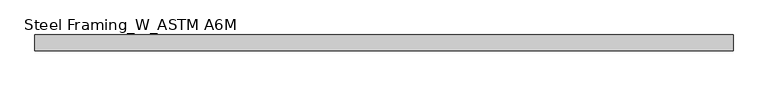
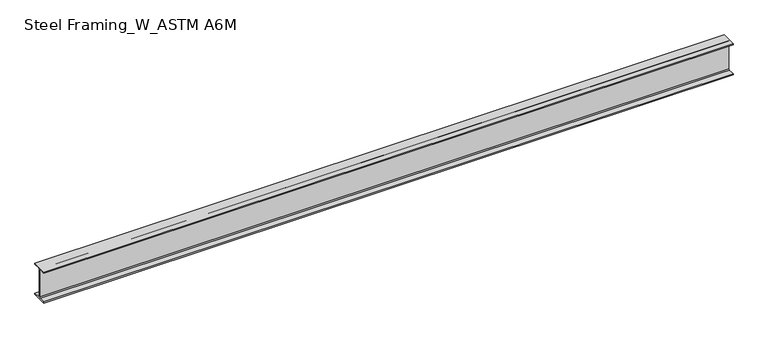
"""IFC4 building model written with IfcOpenShell, lengths in millimetres: beam geometry, Steel Framing_W_ASTM A6M : H_SB_AR_S02_W360x51_RG1."""

import ifcopenshell
import ifcopenshell.guid

model = None  # the IFC model being written
_history = None  # IfcOwnerHistory: only IFC2X3 demands one
_inside = {}  # id of a spatial element -> (the spatial element, [elements in it])
_under = {}  # id of a project, library or spatial element -> (it, [spatial elements below it])
_declared = {}  # id of a project -> (the project, [libraries it declares])
_typed = {}  # id of a type object -> (the type object, [elements of that type])
_made_of = {}  # id of a material, layer set ... -> (it, [elements and type objects made of it])


def new_model(schema):
    """Start an empty IFC model of exactly this schema.

    Asked for "IFC4X3", IfcOpenShell would pick the latest addendum, in which some entities
    have other attributes; the version numbers below select the first issue.
    IFC2X3 requires an IfcOwnerHistory on every rooted entity: one is made here for all.
    """
    global model, _history
    if schema == "IFC4X3":
        model = ifcopenshell.file(schema_version=(4, 3, 0, 0))
    else:
        model = ifcopenshell.file(schema=schema)
    _inside.clear()
    _under.clear()
    _declared.clear()
    _typed.clear()
    _made_of.clear()
    _history = None
    if model.schema == "IFC2X3":
        org = make("IfcOrganization", Name="unknown")
        user = make(
            "IfcPersonAndOrganization",
            ThePerson=make("IfcPerson", FamilyName="unknown"),
            TheOrganization=org,
        )
        app = make(
            "IfcApplication",
            ApplicationDeveloper=org,
            Version="unknown",
            ApplicationFullName="unknown",
            ApplicationIdentifier="unknown",
        )
        _history = make(
            "IfcOwnerHistory",
            OwningUser=user,
            OwningApplication=app,
            ChangeAction="ADDED",
            CreationDate=0,
        )
    return model


def make(cls, **values):
    """One entity of the class cls with the attributes given. An attribute that is None is left unset."""
    return model.create_entity(
        cls, **{name: value for name, value in values.items() if value is not None}
    )


def rooted(cls, **values):
    """An entity with a GlobalId (a new one), such as an element, a storey or a relation."""
    return make(cls, GlobalId=ifcopenshell.guid.new(), OwnerHistory=_history, **values)


def si_unit(unit_type, name, prefix=None):
    """IfcSIUnit, for example si_unit("LENGTHUNIT", "METRE", prefix="MILLI")."""
    return make("IfcSIUnit", UnitType=unit_type, Prefix=prefix, Name=name)


def assignment(units):
    """IfcUnitAssignment: the units of a project."""
    return None if units is None else make("IfcUnitAssignment", Units=units)


def point(xyz):
    """IfcCartesianPoint."""
    return None if xyz is None else make("IfcCartesianPoint", Coordinates=xyz)


def direction(xyz):
    """IfcDirection."""
    return None if xyz is None else make("IfcDirection", DirectionRatios=xyz)


def frame(location, z_axis=None, x_axis=None):
    """IfcAxis2Placement3D, a coordinate frame: its origin and axes. An axis left out is left unset."""
    return make(
        "IfcAxis2Placement3D",
        Location=point(location),
        Axis=direction(z_axis),
        RefDirection=direction(x_axis),
    )


def frame_2d(location, x_axis=None):
    """IfcAxis2Placement2D, a coordinate frame in the plane: its origin and x axis."""
    return make(
        "IfcAxis2Placement2D", Location=point(location), RefDirection=direction(x_axis)
    )


def origin():
    """The frame at (0, 0, 0) with its axes left unset."""
    return frame((0.0, 0.0, 0.0))


def place(relative_to, where):
    """IfcLocalPlacement: puts the frame where relative to a parent placement (None: the world)."""
    return make(
        "IfcLocalPlacement", PlacementRelTo=relative_to, RelativePlacement=where
    )


def context(
    kind, dimensions, precision=None, world=None, true_north=None, identifier=None
):
    """IfcGeometricRepresentationContext, for example the 3D "Model" context."""
    return make(
        "IfcGeometricRepresentationContext",
        ContextIdentifier=identifier,
        ContextType=kind,
        CoordinateSpaceDimension=dimensions,
        Precision=precision,
        WorldCoordinateSystem=world,
        TrueNorth=true_north,
    )


def project(units=None, contexts=None):
    """IfcProject with its units and contexts."""
    return rooted(
        "IfcProject",
        Name="project",
        RepresentationContexts=contexts,
        UnitsInContext=assignment(units),
    )


def spatial(cls, under=None, at=None, **own):
    """A site, building, storey or space (cls), placed at a placement, below another one or the project."""
    s = rooted(cls, ObjectPlacement=at, **own)
    if under is not None:
        _under.setdefault(under.id(), (under, []))[1].append(s)
    return s


def polyline(points):
    """IfcPolyline through the points."""
    return make("IfcPolyline", Points=[point(p) for p in points])


def circle_curve(where, radius):
    """IfcCircle in the frame where."""
    return make("IfcCircle", Position=where, Radius=radius)


def trimmed(basis, trim1, trim2, sense, master):
    """IfcTrimmedCurve: the piece of a basis curve between two trims."""
    return make(
        "IfcTrimmedCurve",
        BasisCurve=basis,
        Trim1=trim1,
        Trim2=trim2,
        SenseAgreement=sense,
        MasterRepresentation=master,
    )


def segment(curve, same_sense, transition):
    """IfcCompositeCurveSegment."""
    return make(
        "IfcCompositeCurveSegment",
        Transition=transition,
        SameSense=same_sense,
        ParentCurve=curve,
    )


def composite_curve(segments, self_intersect=None):
    """IfcCompositeCurve: segments joined end to end."""
    return make("IfcCompositeCurve", Segments=segments, SelfIntersect=self_intersect)


def outline(outer, holes=None, kind="AREA"):
    """IfcArbitraryClosedProfileDef: a profile drawn as a closed curve; with holes, ...WithVoids."""
    if holes is None:
        return make("IfcArbitraryClosedProfileDef", ProfileType=kind, OuterCurve=outer)
    return make(
        "IfcArbitraryProfileDefWithVoids",
        ProfileType=kind,
        OuterCurve=outer,
        InnerCurves=holes,
    )


def extrude(swept, where, along, depth):
    """IfcExtrudedAreaSolid: the profile swept, set in the frame where, extruded along a direction by depth."""
    return make(
        "IfcExtrudedAreaSolid",
        SweptArea=swept,
        Position=where,
        ExtrudedDirection=direction(along),
        Depth=depth,
    )


def shape(context_of_items, identifier, shape_type, items):
    """IfcShapeRepresentation: the items that make up one representation, for example the "Body"."""
    return make(
        "IfcShapeRepresentation",
        ContextOfItems=context_of_items,
        RepresentationIdentifier=identifier,
        RepresentationType=shape_type,
        Items=items,
    )


def source(mapping_origin, context_of_items, identifier, shape_type, items):
    """IfcRepresentationMap: a shape defined once, which mapped items show again and again."""
    return make(
        "IfcRepresentationMap",
        MappingOrigin=mapping_origin,
        MappedRepresentation=shape(context_of_items, identifier, shape_type, items),
    )


def transform(
    local_origin,
    x_axis=None,
    y_axis=None,
    z_axis=None,
    scale=None,
    scale2=None,
    scale3=None,
    uniform=True,
):
    """IfcCartesianTransformationOperator3D, or its non-uniform kind. x_axis, y_axis, z_axis: its Axis1, 2, 3."""
    if uniform:
        return make(
            "IfcCartesianTransformationOperator3D",
            Axis1=direction(x_axis),
            Axis2=direction(y_axis),
            LocalOrigin=point(local_origin),
            Scale=scale,
            Axis3=direction(z_axis),
        )
    return make(
        "IfcCartesianTransformationOperator3DnonUniform",
        Axis1=direction(x_axis),
        Axis2=direction(y_axis),
        LocalOrigin=point(local_origin),
        Scale=scale,
        Axis3=direction(z_axis),
        Scale2=scale2,
        Scale3=scale3,
    )


def mapped(mapping_source, mapping_target):
    """IfcMappedItem: shows the shape of a source again, moved by a transform."""
    return make(
        "IfcMappedItem", MappingSource=mapping_source, MappingTarget=mapping_target
    )


def made_of(thing, what):
    """Note that an element or type object is made of a material, layer set ...; save() writes the relation."""
    if what is not None:
        _made_of.setdefault(what.id(), (what, []))[1].append(thing)
    return thing


def element(
    cls,
    number,
    at=None,
    inside=None,
    cuts=None,
    type_object=None,
    material=None,
    context=None,
    identifier="Body",
    shape_type=None,
    held_by="IfcProductDefinitionShape",
    body=None,
    shapes=None,
    **own,
):
    """One element of the class cls, such as IfcWall. Its Tag is "e" and its number.

    at: its placement. inside: the storey or other place that contains it. cuts: it is an
    opening in that element (IfcRelVoidsElement). A single representation is given by context,
    identifier, shape_type and body (its items); several are given by shapes. held_by: the class
    of the entity that holds the representations. save() writes the other relations.
    """
    e = rooted(cls, Tag="e%d" % number, ObjectPlacement=at, **own)
    if body is not None:
        shapes = [shape(context, identifier, shape_type, body)]
    if shapes is not None:
        e.Representation = make(held_by, Representations=shapes)
    if inside is not None:
        _inside.setdefault(inside.id(), (inside, []))[1].append(e)
    if cuts is not None:
        rooted(
            "IfcRelVoidsElement", RelatingBuildingElement=cuts, RelatedOpeningElement=e
        )
    if type_object is not None:
        _typed.setdefault(type_object.id(), (type_object, []))[1].append(e)
    return made_of(e, material)


def aggregate(whole, parts):
    """IfcRelAggregates: a whole, such as a stair, and the parts it consists of."""
    return rooted("IfcRelAggregates", RelatingObject=whole, RelatedObjects=parts)


def save(model, path):
    """Write the relations noted so far, then the file.

    IfcRelAggregates (storeys below a building ...), IfcRelContainedInSpatialStructure (elements
    in a storey), IfcRelDefinesByType, IfcRelAssociatesMaterial and IfcRelDeclares: one each for
    every whole, place, type object, material and project.
    """
    for whole, parts in _under.values():
        aggregate(whole, parts)
    for where, things in _inside.values():
        rooted(
            "IfcRelContainedInSpatialStructure",
            RelatedElements=things,
            RelatingStructure=where,
        )
    for kind, things in _typed.values():
        rooted("IfcRelDefinesByType", RelatedObjects=things, RelatingType=kind)
    for what, things in _made_of.values():
        rooted("IfcRelAssociatesMaterial", RelatedObjects=things, RelatingMaterial=what)
    for by, libraries in _declared.values():
        rooted("IfcRelDeclares", RelatingContext=by, RelatedDefinitions=libraries)
    model.write(path)


def steel_framing_w_astm_a6m_b27ce7d5(model_context):
    return source(origin(), model_context, "Body", "SweptSolid", [
        extrude(outline(composite_curve([segment(polyline([(85.5, -166.4), (85.5, -178.0), (-85.5, -178.0), (-85.5, -166.4), (-13.72, -166.4)]), True, "CONTINUOUS"), segment(trimmed(circle_curve(frame_2d((-13.72, -156.3)), 10.1), [point((-13.72, -166.4))], [point((-3.62, -156.3))], True, "CARTESIAN"), True, "CONTINUOUS"), segment(polyline([(-3.62, -156.3), (-3.62, 156.3)]), True, "CONTINUOUS"), segment(trimmed(circle_curve(frame_2d((-13.72, 156.3)), 10.1), [point((-3.62, 156.3))], [point((-13.72, 166.4))], True, "CARTESIAN"), True, "CONTINUOUS"), segment(polyline([(-13.72, 166.4), (-85.5, 166.4), (-85.5, 178.0), (85.5, 178.0), (85.5, 166.4), (13.72, 166.4)]), True, "CONTINUOUS"), segment(trimmed(circle_curve(frame_2d((13.72, 156.3)), 10.1), [point((13.72, 166.4))], [point((3.62, 156.3))], True, "CARTESIAN"), True, "CONTINUOUS"), segment(polyline([(3.62, 156.3), (3.62, -156.3)]), True, "CONTINUOUS"), segment(trimmed(circle_curve(frame_2d((13.72, -156.3)), 10.1), [point((3.62, -156.3))], [point((13.72, -166.4))], True, "CARTESIAN"), True, "CONTINUOUS"), segment(polyline([(13.72, -166.4), (85.5, -166.4)]), True, "CONTINUOUS")], self_intersect=False)), frame((-3736.95, 0.0, 0.0), z_axis=(1.0, 0.0, 0.0), x_axis=(0.0, 1.0, 0.0)), (0.0, 0.0, 1.0), 7511.8),
    ])


if __name__ == "__main__":
    model = new_model("IFC4")
    model_context = context("Model", 3, world=origin())
    ifc_project = project(units=[si_unit("LENGTHUNIT", "METRE", prefix="MILLI")], contexts=[model_context])
    site = spatial("IfcSite", under=ifc_project)
    building = spatial("IfcBuilding", under=site)
    placement = place(None, origin())
    steel_framing_w_astm_a6m_shape = steel_framing_w_astm_a6m_b27ce7d5(model_context)
    element("IfcBeam", 1, ObjectType="Steel Framing_W_ASTM A6M : H_SB_AR_S02_W360x51_RG1", at=placement, inside=building, context=model_context, shape_type="MappedRepresentation", body=[
        mapped(steel_framing_w_astm_a6m_shape, transform((0.0, 0.0, 0.0), x_axis=(1.0, 0.0, 0.0), y_axis=(0.0, 1.0, 0.0), z_axis=(0.0, 0.0, 1.0))),
    ])
    save(model, "model.ifc")

# Revit data of these elements
# Type "Steel Framing_W_ASTM A6M : H_SB_AR_S02_W360x51_RG1"
#   Section Name Key = "W14x34"
#   Width = 17.1 cm
#   Web Thickness = 0.724 cm
#   Web Fillet = 1.01 cm
#   Warping Constant = 287000.0 cm⁶
#   Torsional Moment of Inertia = 23.70 cm⁴
#   Section Area = 64.5 cm²
#   Plastic Modulus weak axis = 174.0 cm³
#   Plastic Modulus strong axis = 895.0 cm³
#   Perimeter = 1.36 m²/m
#   Nominal Weight = 51.00 kgf/m
#   Moment of Inertia weak axis = 970.00 cm⁴
#   Moment of Inertia strong axis = 14200.00 cm⁴
#   Height = 35.6 cm
#   Flange Thickness = 1.16 cm
#   Elastic Modulus weak axis = 113.0 cm³
#   Elastic Modulus strong axis = 796.0 cm³
#   Centroid Vertical = 17.8 cm
#   Centroid Horizontal = 8.55 cm
#   Length [instance default] = 1500 mm
#   Structural Material [instance default] = Steel, 45-345
#   Bolt Spacing = 0
#   Assembly Code = ""
# Element 1 (IfcBeam, "Steel Framing_W_ASTM A6M : H_SB_AR_S02_W360x51_RG1")
#   Materials on its faces: "Steel, 45-345"
# Materials
#   "Steel, 45-345": class "Metal", colour RGB 189 187 185, transparency 0, Description = "Steel 345 MPa", Cost = 0
